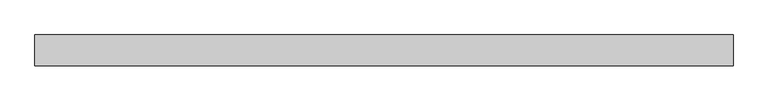
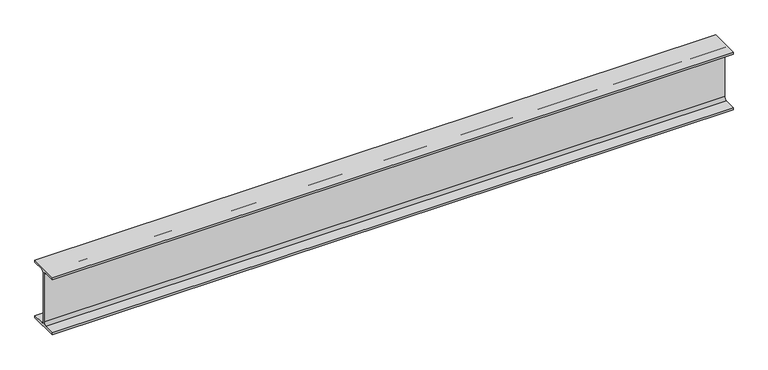
"""IFC4 building model written with IfcOpenShell, lengths in millimetres: beam geometry, 0912_Steel Framing_H-KSD3502 : H_SB_ASB_H-250x125x6x9."""

from ifc_helpers import new_model, si_unit, point, frame, frame_2d, origin, place, context, project, spatial, polyline, circle_curve, trimmed, segment, composite_curve, outline, extrude, source, transform, mapped, element, save


def beam_c8a320e1(model_context):
    return source(origin(), model_context, "Body", "SweptSolid", [
        extrude(outline(composite_curve([segment(polyline([(62.5, -116.0), (62.5, -125.0), (-62.5, -125.0), (-62.5, -116.0), (-15.0, -116.0)]), True, "CONTINUOUS"), segment(trimmed(circle_curve(frame_2d((-15.0, -104.0)), 12.0), [point((-15.0, -116.0))], [point((-3.0, -104.0))], True, "CARTESIAN"), True, "CONTINUOUS"), segment(polyline([(-3.0, -104.0), (-3.0, 104.0)]), True, "CONTINUOUS"), segment(trimmed(circle_curve(frame_2d((-15.0, 104.0)), 12.0), [point((-3.0, 104.0))], [point((-15.0, 116.0))], True, "CARTESIAN"), True, "CONTINUOUS"), segment(polyline([(-15.0, 116.0), (-62.5, 116.0), (-62.5, 125.0), (62.5, 125.0), (62.5, 116.0), (15.0, 116.0)]), True, "CONTINUOUS"), segment(trimmed(circle_curve(frame_2d((15.0, 104.0)), 12.0), [point((15.0, 116.0))], [point((3.0, 104.0))], True, "CARTESIAN"), True, "CONTINUOUS"), segment(polyline([(3.0, 104.0), (3.0, -104.0)]), True, "CONTINUOUS"), segment(trimmed(circle_curve(frame_2d((15.0, -104.0)), 12.0), [point((3.0, -104.0))], [point((15.0, -116.0))], True, "CARTESIAN"), True, "CONTINUOUS"), segment(polyline([(15.0, -116.0), (62.5, -116.0)]), True, "CONTINUOUS")], self_intersect=False)), frame((-1404.8, 0.0, 0.0), z_axis=(1.0, 0.0, 0.0), x_axis=(0.0, 1.0, 0.0)), (0.0, 0.0, 1.0), 2809.6),
    ])


if __name__ == "__main__":
    model = new_model("IFC4")
    model_context = context("Model", 3, world=origin())
    ifc_project = project(units=[si_unit("LENGTHUNIT", "METRE", prefix="MILLI")], contexts=[model_context])
    site = spatial("IfcSite", under=ifc_project)
    building = spatial("IfcBuilding", under=site)
    placement = place(None, origin())
    beam_shape = beam_c8a320e1(model_context)
    element("IfcBeam", 1, ObjectType="0912_Steel Framing_H-KSD3502 : H_SB_ASB_H-250x125x6x9", at=placement, inside=building, context=model_context, shape_type="MappedRepresentation", body=[
        mapped(beam_shape, transform((0.0, 0.0, 0.0), x_axis=(1.0, 0.0, 0.0), y_axis=(0.0, 1.0, 0.0), z_axis=(0.0, 0.0, 1.0))),
    ])
    save(model, "model.ifc")

# Revit data of these elements
# Type "0912_Steel Framing_H-KSD3502 : H_SB_ASB_H-250x125x6x9"
#   H_WM Code_1 = "S01AA003-00001 | Main Steel Structure Fabrication Work | Shelter/Building | Light Steel - Standard (30KG/M>Weight) | Material: (   )"
#   H_WM Code_2 = "S03AA029-00001 | Main Steel Structure Erection Work | Shelter/Building | Light Steel (30KG/M>Weight) | Material: (   )"
#   H_WM Code_3 = "S01AA010-00001 | Main Steel Structure Fabrication Work | Shelter/Building | Steel Painting/Coating | for Non-Fireproofed Steel Surface, Surface Preparation, Primer, Second & Final Coat | Material: (   )"
#   H_Q'ty Cal Type Tag = "SB-Q2"
#   Width = 12.5 cm
#   Web Thickness = 0.6 cm
#   Web Fillet = 1.2 cm
#   Warping Constant = 42539.8 cm⁶
#   W = 0
#   Torsional Moment of Inertia = 7.8102 cm⁴
#   Section Area = 37.66 cm²
#   Plastic Modulus weak axis = 73.1 cm³
#   Plastic Modulus strong axis = 366.0 cm³
#   Perimeter = 0.97 m²/m
#   Nominal Weight = 29.60 kgf/m
#   Moment of Inertia weak axis = 294.00 cm⁴
#   Moment of Inertia strong axis = 4050.00 cm⁴
#   Height = 25.0 cm
#   Flange Thickness = 0.9 cm
#   Elastic Modulus weak axis = 47.0 cm³
#   Elastic Modulus strong axis = 324.0 cm³
#   Centroid Vertical = 12.5 cm
#   Centroid Horizontal = 6.25 cm
#   Ix = 40500000
#   Length [instance default] = 1.5240 m
#   Zx = 366000
#   b = 0.1250 m
#   h = 0.2500 m
#   r = 0.0120 m
#   s = 0.0060 m
#   t = 0.0090 m
#   A = 0.003766 m²
#   Structural Material [instance default] = Steel, 45-345
#   Assembly Code = ""
# Element 1 (IfcBeam, "0912_Steel Framing_H-KSD3502 : H_SB_ASB_H-250x125x6x9")
#   Structural Material = none
# Materials
#   "Steel, 45-345": class "Metal", colour RGB 189 187 185, transparency 0, Description = "Steel 345 MPa", Cost = 0
